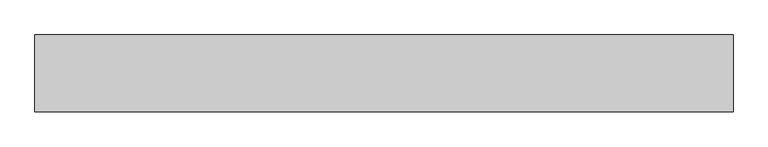
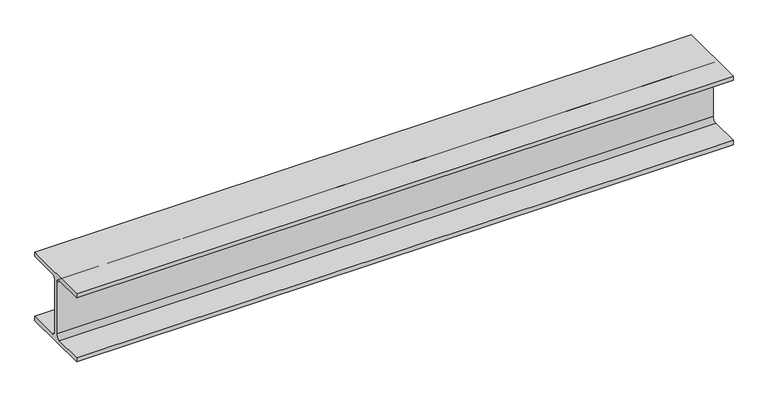
"""IFC4 building model written with IfcOpenShell, lengths in millimetres: beam geometry, 0912_Steel Framing_H-KSD3502 : H_SB_ASB_H-200x200x8x12."""

import ifcopenshell
import ifcopenshell.guid

model = None  # the IFC model being written
_history = None  # IfcOwnerHistory: only IFC2X3 demands one
_inside = {}  # id of a spatial element -> (the spatial element, [elements in it])
_under = {}  # id of a project, library or spatial element -> (it, [spatial elements below it])
_declared = {}  # id of a project -> (the project, [libraries it declares])
_typed = {}  # id of a type object -> (the type object, [elements of that type])
_made_of = {}  # id of a material, layer set ... -> (it, [elements and type objects made of it])


def new_model(schema):
    """Start an empty IFC model of exactly this schema.

    Asked for "IFC4X3", IfcOpenShell would pick the latest addendum, in which some entities
    have other attributes; the version numbers below select the first issue.
    IFC2X3 requires an IfcOwnerHistory on every rooted entity: one is made here for all.
    """
    global model, _history
    if schema == "IFC4X3":
        model = ifcopenshell.file(schema_version=(4, 3, 0, 0))
    else:
        model = ifcopenshell.file(schema=schema)
    _inside.clear()
    _under.clear()
    _declared.clear()
    _typed.clear()
    _made_of.clear()
    _history = None
    if model.schema == "IFC2X3":
        org = make("IfcOrganization", Name="unknown")
        user = make(
            "IfcPersonAndOrganization",
            ThePerson=make("IfcPerson", FamilyName="unknown"),
            TheOrganization=org,
        )
        app = make(
            "IfcApplication",
            ApplicationDeveloper=org,
            Version="unknown",
            ApplicationFullName="unknown",
            ApplicationIdentifier="unknown",
        )
        _history = make(
            "IfcOwnerHistory",
            OwningUser=user,
            OwningApplication=app,
            ChangeAction="ADDED",
            CreationDate=0,
        )
    return model


def make(cls, **values):
    """One entity of the class cls with the attributes given. An attribute that is None is left unset."""
    return model.create_entity(
        cls, **{name: value for name, value in values.items() if value is not None}
    )


def rooted(cls, **values):
    """An entity with a GlobalId (a new one), such as an element, a storey or a relation."""
    return make(cls, GlobalId=ifcopenshell.guid.new(), OwnerHistory=_history, **values)


def si_unit(unit_type, name, prefix=None):
    """IfcSIUnit, for example si_unit("LENGTHUNIT", "METRE", prefix="MILLI")."""
    return make("IfcSIUnit", UnitType=unit_type, Prefix=prefix, Name=name)


def assignment(units):
    """IfcUnitAssignment: the units of a project."""
    return None if units is None else make("IfcUnitAssignment", Units=units)


def point(xyz):
    """IfcCartesianPoint."""
    return None if xyz is None else make("IfcCartesianPoint", Coordinates=xyz)


def direction(xyz):
    """IfcDirection."""
    return None if xyz is None else make("IfcDirection", DirectionRatios=xyz)


def frame(location, z_axis=None, x_axis=None):
    """IfcAxis2Placement3D, a coordinate frame: its origin and axes. An axis left out is left unset."""
    return make(
        "IfcAxis2Placement3D",
        Location=point(location),
        Axis=direction(z_axis),
        RefDirection=direction(x_axis),
    )


def frame_2d(location, x_axis=None):
    """IfcAxis2Placement2D, a coordinate frame in the plane: its origin and x axis."""
    return make(
        "IfcAxis2Placement2D", Location=point(location), RefDirection=direction(x_axis)
    )


def origin():
    """The frame at (0, 0, 0) with its axes left unset."""
    return frame((0.0, 0.0, 0.0))


def place(relative_to, where):
    """IfcLocalPlacement: puts the frame where relative to a parent placement (None: the world)."""
    return make(
        "IfcLocalPlacement", PlacementRelTo=relative_to, RelativePlacement=where
    )


def context(
    kind, dimensions, precision=None, world=None, true_north=None, identifier=None
):
    """IfcGeometricRepresentationContext, for example the 3D "Model" context."""
    return make(
        "IfcGeometricRepresentationContext",
        ContextIdentifier=identifier,
        ContextType=kind,
        CoordinateSpaceDimension=dimensions,
        Precision=precision,
        WorldCoordinateSystem=world,
        TrueNorth=true_north,
    )


def project(units=None, contexts=None):
    """IfcProject with its units and contexts."""
    return rooted(
        "IfcProject",
        Name="project",
        RepresentationContexts=contexts,
        UnitsInContext=assignment(units),
    )


def spatial(cls, under=None, at=None, **own):
    """A site, building, storey or space (cls), placed at a placement, below another one or the project."""
    s = rooted(cls, ObjectPlacement=at, **own)
    if under is not None:
        _under.setdefault(under.id(), (under, []))[1].append(s)
    return s


def polyline(points):
    """IfcPolyline through the points."""
    return make("IfcPolyline", Points=[point(p) for p in points])


def circle_curve(where, radius):
    """IfcCircle in the frame where."""
    return make("IfcCircle", Position=where, Radius=radius)


def trimmed(basis, trim1, trim2, sense, master):
    """IfcTrimmedCurve: the piece of a basis curve between two trims."""
    return make(
        "IfcTrimmedCurve",
        BasisCurve=basis,
        Trim1=trim1,
        Trim2=trim2,
        SenseAgreement=sense,
        MasterRepresentation=master,
    )


def segment(curve, same_sense, transition):
    """IfcCompositeCurveSegment."""
    return make(
        "IfcCompositeCurveSegment",
        Transition=transition,
        SameSense=same_sense,
        ParentCurve=curve,
    )


def composite_curve(segments, self_intersect=None):
    """IfcCompositeCurve: segments joined end to end."""
    return make("IfcCompositeCurve", Segments=segments, SelfIntersect=self_intersect)


def outline(outer, holes=None, kind="AREA"):
    """IfcArbitraryClosedProfileDef: a profile drawn as a closed curve; with holes, ...WithVoids."""
    if holes is None:
        return make("IfcArbitraryClosedProfileDef", ProfileType=kind, OuterCurve=outer)
    return make(
        "IfcArbitraryProfileDefWithVoids",
        ProfileType=kind,
        OuterCurve=outer,
        InnerCurves=holes,
    )


def extrude(swept, where, along, depth):
    """IfcExtrudedAreaSolid: the profile swept, set in the frame where, extruded along a direction by depth."""
    return make(
        "IfcExtrudedAreaSolid",
        SweptArea=swept,
        Position=where,
        ExtrudedDirection=direction(along),
        Depth=depth,
    )


def shape(context_of_items, identifier, shape_type, items):
    """IfcShapeRepresentation: the items that make up one representation, for example the "Body"."""
    return make(
        "IfcShapeRepresentation",
        ContextOfItems=context_of_items,
        RepresentationIdentifier=identifier,
        RepresentationType=shape_type,
        Items=items,
    )


def source(mapping_origin, context_of_items, identifier, shape_type, items):
    """IfcRepresentationMap: a shape defined once, which mapped items show again and again."""
    return make(
        "IfcRepresentationMap",
        MappingOrigin=mapping_origin,
        MappedRepresentation=shape(context_of_items, identifier, shape_type, items),
    )


def transform(
    local_origin,
    x_axis=None,
    y_axis=None,
    z_axis=None,
    scale=None,
    scale2=None,
    scale3=None,
    uniform=True,
):
    """IfcCartesianTransformationOperator3D, or its non-uniform kind. x_axis, y_axis, z_axis: its Axis1, 2, 3."""
    if uniform:
        return make(
            "IfcCartesianTransformationOperator3D",
            Axis1=direction(x_axis),
            Axis2=direction(y_axis),
            LocalOrigin=point(local_origin),
            Scale=scale,
            Axis3=direction(z_axis),
        )
    return make(
        "IfcCartesianTransformationOperator3DnonUniform",
        Axis1=direction(x_axis),
        Axis2=direction(y_axis),
        LocalOrigin=point(local_origin),
        Scale=scale,
        Axis3=direction(z_axis),
        Scale2=scale2,
        Scale3=scale3,
    )


def mapped(mapping_source, mapping_target):
    """IfcMappedItem: shows the shape of a source again, moved by a transform."""
    return make(
        "IfcMappedItem", MappingSource=mapping_source, MappingTarget=mapping_target
    )


def made_of(thing, what):
    """Note that an element or type object is made of a material, layer set ...; save() writes the relation."""
    if what is not None:
        _made_of.setdefault(what.id(), (what, []))[1].append(thing)
    return thing


def element(
    cls,
    number,
    at=None,
    inside=None,
    cuts=None,
    type_object=None,
    material=None,
    context=None,
    identifier="Body",
    shape_type=None,
    held_by="IfcProductDefinitionShape",
    body=None,
    shapes=None,
    **own,
):
    """One element of the class cls, such as IfcWall. Its Tag is "e" and its number.

    at: its placement. inside: the storey or other place that contains it. cuts: it is an
    opening in that element (IfcRelVoidsElement). A single representation is given by context,
    identifier, shape_type and body (its items); several are given by shapes. held_by: the class
    of the entity that holds the representations. save() writes the other relations.
    """
    e = rooted(cls, Tag="e%d" % number, ObjectPlacement=at, **own)
    if body is not None:
        shapes = [shape(context, identifier, shape_type, body)]
    if shapes is not None:
        e.Representation = make(held_by, Representations=shapes)
    if inside is not None:
        _inside.setdefault(inside.id(), (inside, []))[1].append(e)
    if cuts is not None:
        rooted(
            "IfcRelVoidsElement", RelatingBuildingElement=cuts, RelatedOpeningElement=e
        )
    if type_object is not None:
        _typed.setdefault(type_object.id(), (type_object, []))[1].append(e)
    return made_of(e, material)


def aggregate(whole, parts):
    """IfcRelAggregates: a whole, such as a stair, and the parts it consists of."""
    return rooted("IfcRelAggregates", RelatingObject=whole, RelatedObjects=parts)


def save(model, path):
    """Write the relations noted so far, then the file.

    IfcRelAggregates (storeys below a building ...), IfcRelContainedInSpatialStructure (elements
    in a storey), IfcRelDefinesByType, IfcRelAssociatesMaterial and IfcRelDeclares: one each for
    every whole, place, type object, material and project.
    """
    for whole, parts in _under.values():
        aggregate(whole, parts)
    for where, things in _inside.values():
        rooted(
            "IfcRelContainedInSpatialStructure",
            RelatedElements=things,
            RelatingStructure=where,
        )
    for kind, things in _typed.values():
        rooted("IfcRelDefinesByType", RelatedObjects=things, RelatingType=kind)
    for what, things in _made_of.values():
        rooted("IfcRelAssociatesMaterial", RelatedObjects=things, RelatingMaterial=what)
    for by, libraries in _declared.values():
        rooted("IfcRelDeclares", RelatingContext=by, RelatedDefinitions=libraries)
    model.write(path)


def beam_45f125b0(model_context):
    return source(origin(), model_context, "Body", "SweptSolid", [
        extrude(outline(composite_curve([segment(polyline([(100.0, -88.0), (100.0, -100.0), (-100.0, -100.0), (-100.0, -88.0), (-17.0, -88.0)]), True, "CONTINUOUS"), segment(trimmed(circle_curve(frame_2d((-17.0, -75.0)), 13.0), [point((-17.0, -88.0))], [point((-4.0, -75.0))], True, "CARTESIAN"), True, "CONTINUOUS"), segment(polyline([(-4.0, -75.0), (-4.0, 75.0)]), True, "CONTINUOUS"), segment(trimmed(circle_curve(frame_2d((-17.0, 75.0)), 13.0), [point((-4.0, 75.0))], [point((-17.0, 88.0))], True, "CARTESIAN"), True, "CONTINUOUS"), segment(polyline([(-17.0, 88.0), (-100.0, 88.0), (-100.0, 100.0), (100.0, 100.0), (100.0, 88.0), (17.0, 88.0)]), True, "CONTINUOUS"), segment(trimmed(circle_curve(frame_2d((17.0, 75.0)), 13.0), [point((17.0, 88.0))], [point((4.0, 75.0))], True, "CARTESIAN"), True, "CONTINUOUS"), segment(polyline([(4.0, 75.0), (4.0, -75.0)]), True, "CONTINUOUS"), segment(trimmed(circle_curve(frame_2d((17.0, -75.0)), 13.0), [point((4.0, -75.0))], [point((17.0, -88.0))], True, "CARTESIAN"), True, "CONTINUOUS"), segment(polyline([(17.0, -88.0), (100.0, -88.0)]), True, "CONTINUOUS")], self_intersect=False)), frame((-1035.0333333, 0.0, 0.0), z_axis=(1.0, 0.0, 0.0), x_axis=(0.0, 1.0, 0.0)), (0.0, 0.0, 1.0), 1820.0666667),
    ])


if __name__ == "__main__":
    model = new_model("IFC4")
    model_context = context("Model", 3, world=origin())
    ifc_project = project(units=[si_unit("LENGTHUNIT", "METRE", prefix="MILLI")], contexts=[model_context])
    site = spatial("IfcSite", under=ifc_project)
    building = spatial("IfcBuilding", under=site)
    placement = place(None, origin())
    beam_shape = beam_45f125b0(model_context)
    element("IfcBeam", 1, ObjectType="0912_Steel Framing_H-KSD3502 : H_SB_ASB_H-200x200x8x12", at=placement, inside=building, context=model_context, shape_type="MappedRepresentation", body=[
        mapped(beam_shape, transform((0.0, 0.0, 0.0), x_axis=(1.0, 0.0, 0.0), y_axis=(0.0, 1.0, 0.0), z_axis=(0.0, 0.0, 1.0))),
    ])
    save(model, "model.ifc")

# Revit data of these elements
# Type "0912_Steel Framing_H-KSD3502 : H_SB_ASB_H-200x200x8x12"
#   H_WM Code_1 = "S01AA002-00001 | Main Steel Structure Fabrication Work | Shelter/Building | Medium Steel - Standard (90KG/M>Weight≥30KG/M) | Material: (   )"
#   H_WM Code_2 = "S03AA028-00001 | Main Steel Structure Erection Work | Shelter/Building | Medium Steel (90KG/M>Weight≥30KG/M) | Material: (   )"
#   H_WM Code_3 = "S01AA010-00001 | Main Steel Structure Fabrication Work | Shelter/Building | Steel Painting/Coating | for Non-Fireproofed Steel Surface, Surface Preparation, Primer, Second & Final Coat | Material: (   )"
#   H_Q'ty Cal Type Tag = "SB-Q2"
#   Width = 20.0 cm
#   Web Thickness = 0.8 cm
#   Web Fillet = 1.3 cm
#   Warping Constant = 141000.0 cm⁶
#   W = 0
#   Torsional Moment of Inertia = 26.2485 cm⁴
#   Section Area = 63.53 cm²
#   Plastic Modulus weak axis = 244.0 cm³
#   Plastic Modulus strong axis = 525.0 cm³
#   Perimeter = 1.16 m²/m
#   Nominal Weight = 49.90 kgf/m
#   Moment of Inertia weak axis = 1600.00 cm⁴
#   Moment of Inertia strong axis = 4720.00 cm⁴
#   Height = 20.0 cm
#   Flange Thickness = 1.2 cm
#   Elastic Modulus weak axis = 160.0 cm³
#   Elastic Modulus strong axis = 472.0 cm³
#   Centroid Vertical = 10.0 cm
#   Centroid Horizontal = 10.0 cm
#   Ix = 47200000
#   Length [instance default] = 1.5240 m
#   Zx = 525000
#   b = 0.2000 m
#   h = 0.2000 m
#   r = 0.0130 m
#   s = 0.0080 m
#   t = 0.0120 m
#   A = 0.006353 m²
#   Structural Material [instance default] = Steel, 45-345
#   Assembly Code = ""
# Element 1 (IfcBeam, "0912_Steel Framing_H-KSD3502 : H_SB_ASB_H-200x200x8x12")
#   Structural Material = none
# Materials
#   "Steel, 45-345": class "Metal", colour RGB 189 187 185, transparency 0, Description = "Steel 345 MPa", Cost = 0
